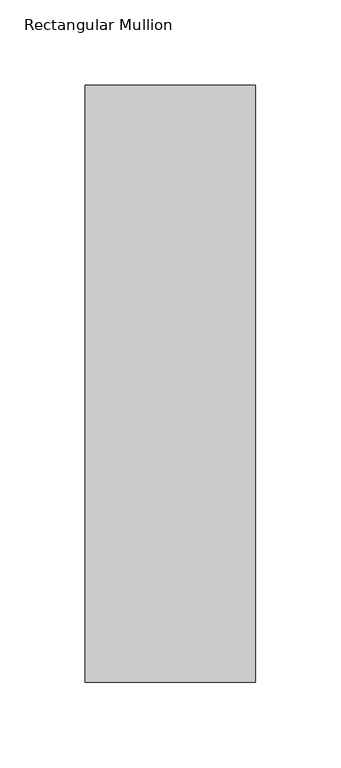
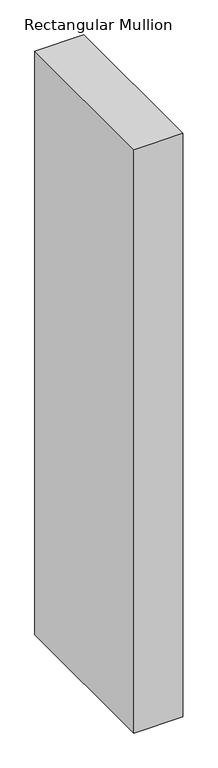
"""IFC4 building model written with IfcOpenShell, lengths in millimetres: member geometry, Rectangular Mullion : WWm-100x350-100mmOffset."""

import ifcopenshell
import ifcopenshell.guid

model = None  # the IFC model being written
_history = None  # IfcOwnerHistory: only IFC2X3 demands one
_inside = {}  # id of a spatial element -> (the spatial element, [elements in it])
_under = {}  # id of a project, library or spatial element -> (it, [spatial elements below it])
_declared = {}  # id of a project -> (the project, [libraries it declares])
_typed = {}  # id of a type object -> (the type object, [elements of that type])
_made_of = {}  # id of a material, layer set ... -> (it, [elements and type objects made of it])


def new_model(schema):
    """Start an empty IFC model of exactly this schema.

    Asked for "IFC4X3", IfcOpenShell would pick the latest addendum, in which some entities
    have other attributes; the version numbers below select the first issue.
    IFC2X3 requires an IfcOwnerHistory on every rooted entity: one is made here for all.
    """
    global model, _history
    if schema == "IFC4X3":
        model = ifcopenshell.file(schema_version=(4, 3, 0, 0))
    else:
        model = ifcopenshell.file(schema=schema)
    _inside.clear()
    _under.clear()
    _declared.clear()
    _typed.clear()
    _made_of.clear()
    _history = None
    if model.schema == "IFC2X3":
        org = make("IfcOrganization", Name="unknown")
        user = make(
            "IfcPersonAndOrganization",
            ThePerson=make("IfcPerson", FamilyName="unknown"),
            TheOrganization=org,
        )
        app = make(
            "IfcApplication",
            ApplicationDeveloper=org,
            Version="unknown",
            ApplicationFullName="unknown",
            ApplicationIdentifier="unknown",
        )
        _history = make(
            "IfcOwnerHistory",
            OwningUser=user,
            OwningApplication=app,
            ChangeAction="ADDED",
            CreationDate=0,
        )
    return model


def make(cls, **values):
    """One entity of the class cls with the attributes given. An attribute that is None is left unset."""
    return model.create_entity(
        cls, **{name: value for name, value in values.items() if value is not None}
    )


def rooted(cls, **values):
    """An entity with a GlobalId (a new one), such as an element, a storey or a relation."""
    return make(cls, GlobalId=ifcopenshell.guid.new(), OwnerHistory=_history, **values)


def si_unit(unit_type, name, prefix=None):
    """IfcSIUnit, for example si_unit("LENGTHUNIT", "METRE", prefix="MILLI")."""
    return make("IfcSIUnit", UnitType=unit_type, Prefix=prefix, Name=name)


def assignment(units):
    """IfcUnitAssignment: the units of a project."""
    return None if units is None else make("IfcUnitAssignment", Units=units)


def point(xyz):
    """IfcCartesianPoint."""
    return None if xyz is None else make("IfcCartesianPoint", Coordinates=xyz)


def direction(xyz):
    """IfcDirection."""
    return None if xyz is None else make("IfcDirection", DirectionRatios=xyz)


def frame(location, z_axis=None, x_axis=None):
    """IfcAxis2Placement3D, a coordinate frame: its origin and axes. An axis left out is left unset."""
    return make(
        "IfcAxis2Placement3D",
        Location=point(location),
        Axis=direction(z_axis),
        RefDirection=direction(x_axis),
    )


def origin():
    """The frame at (0, 0, 0) with its axes left unset."""
    return frame((0.0, 0.0, 0.0))


def place(relative_to, where):
    """IfcLocalPlacement: puts the frame where relative to a parent placement (None: the world)."""
    return make(
        "IfcLocalPlacement", PlacementRelTo=relative_to, RelativePlacement=where
    )


def context(
    kind, dimensions, precision=None, world=None, true_north=None, identifier=None
):
    """IfcGeometricRepresentationContext, for example the 3D "Model" context."""
    return make(
        "IfcGeometricRepresentationContext",
        ContextIdentifier=identifier,
        ContextType=kind,
        CoordinateSpaceDimension=dimensions,
        Precision=precision,
        WorldCoordinateSystem=world,
        TrueNorth=true_north,
    )


def project(units=None, contexts=None):
    """IfcProject with its units and contexts."""
    return rooted(
        "IfcProject",
        Name="project",
        RepresentationContexts=contexts,
        UnitsInContext=assignment(units),
    )


def spatial(cls, under=None, at=None, **own):
    """A site, building, storey or space (cls), placed at a placement, below another one or the project."""
    s = rooted(cls, ObjectPlacement=at, **own)
    if under is not None:
        _under.setdefault(under.id(), (under, []))[1].append(s)
    return s


def polyline(points):
    """IfcPolyline through the points."""
    return make("IfcPolyline", Points=[point(p) for p in points])


def outline(outer, holes=None, kind="AREA"):
    """IfcArbitraryClosedProfileDef: a profile drawn as a closed curve; with holes, ...WithVoids."""
    if holes is None:
        return make("IfcArbitraryClosedProfileDef", ProfileType=kind, OuterCurve=outer)
    return make(
        "IfcArbitraryProfileDefWithVoids",
        ProfileType=kind,
        OuterCurve=outer,
        InnerCurves=holes,
    )


def extrude(swept, where, along, depth):
    """IfcExtrudedAreaSolid: the profile swept, set in the frame where, extruded along a direction by depth."""
    return make(
        "IfcExtrudedAreaSolid",
        SweptArea=swept,
        Position=where,
        ExtrudedDirection=direction(along),
        Depth=depth,
    )


def shape(context_of_items, identifier, shape_type, items):
    """IfcShapeRepresentation: the items that make up one representation, for example the "Body"."""
    return make(
        "IfcShapeRepresentation",
        ContextOfItems=context_of_items,
        RepresentationIdentifier=identifier,
        RepresentationType=shape_type,
        Items=items,
    )


def source(mapping_origin, context_of_items, identifier, shape_type, items):
    """IfcRepresentationMap: a shape defined once, which mapped items show again and again."""
    return make(
        "IfcRepresentationMap",
        MappingOrigin=mapping_origin,
        MappedRepresentation=shape(context_of_items, identifier, shape_type, items),
    )


def transform(
    local_origin,
    x_axis=None,
    y_axis=None,
    z_axis=None,
    scale=None,
    scale2=None,
    scale3=None,
    uniform=True,
):
    """IfcCartesianTransformationOperator3D, or its non-uniform kind. x_axis, y_axis, z_axis: its Axis1, 2, 3."""
    if uniform:
        return make(
            "IfcCartesianTransformationOperator3D",
            Axis1=direction(x_axis),
            Axis2=direction(y_axis),
            LocalOrigin=point(local_origin),
            Scale=scale,
            Axis3=direction(z_axis),
        )
    return make(
        "IfcCartesianTransformationOperator3DnonUniform",
        Axis1=direction(x_axis),
        Axis2=direction(y_axis),
        LocalOrigin=point(local_origin),
        Scale=scale,
        Axis3=direction(z_axis),
        Scale2=scale2,
        Scale3=scale3,
    )


def mapped(mapping_source, mapping_target):
    """IfcMappedItem: shows the shape of a source again, moved by a transform."""
    return make(
        "IfcMappedItem", MappingSource=mapping_source, MappingTarget=mapping_target
    )


def made_of(thing, what):
    """Note that an element or type object is made of a material, layer set ...; save() writes the relation."""
    if what is not None:
        _made_of.setdefault(what.id(), (what, []))[1].append(thing)
    return thing


def element(
    cls,
    number,
    at=None,
    inside=None,
    cuts=None,
    type_object=None,
    material=None,
    context=None,
    identifier="Body",
    shape_type=None,
    held_by="IfcProductDefinitionShape",
    body=None,
    shapes=None,
    **own,
):
    """One element of the class cls, such as IfcWall. Its Tag is "e" and its number.

    at: its placement. inside: the storey or other place that contains it. cuts: it is an
    opening in that element (IfcRelVoidsElement). A single representation is given by context,
    identifier, shape_type and body (its items); several are given by shapes. held_by: the class
    of the entity that holds the representations. save() writes the other relations.
    """
    e = rooted(cls, Tag="e%d" % number, ObjectPlacement=at, **own)
    if body is not None:
        shapes = [shape(context, identifier, shape_type, body)]
    if shapes is not None:
        e.Representation = make(held_by, Representations=shapes)
    if inside is not None:
        _inside.setdefault(inside.id(), (inside, []))[1].append(e)
    if cuts is not None:
        rooted(
            "IfcRelVoidsElement", RelatingBuildingElement=cuts, RelatedOpeningElement=e
        )
    if type_object is not None:
        _typed.setdefault(type_object.id(), (type_object, []))[1].append(e)
    return made_of(e, material)


def aggregate(whole, parts):
    """IfcRelAggregates: a whole, such as a stair, and the parts it consists of."""
    return rooted("IfcRelAggregates", RelatingObject=whole, RelatedObjects=parts)


def save(model, path):
    """Write the relations noted so far, then the file.

    IfcRelAggregates (storeys below a building ...), IfcRelContainedInSpatialStructure (elements
    in a storey), IfcRelDefinesByType, IfcRelAssociatesMaterial and IfcRelDeclares: one each for
    every whole, place, type object, material and project.
    """
    for whole, parts in _under.values():
        aggregate(whole, parts)
    for where, things in _inside.values():
        rooted(
            "IfcRelContainedInSpatialStructure",
            RelatedElements=things,
            RelatingStructure=where,
        )
    for kind, things in _typed.values():
        rooted("IfcRelDefinesByType", RelatedObjects=things, RelatingType=kind)
    for what, things in _made_of.values():
        rooted("IfcRelAssociatesMaterial", RelatedObjects=things, RelatingMaterial=what)
    for by, libraries in _declared.values():
        rooted("IfcRelDeclares", RelatingContext=by, RelatedDefinitions=libraries)
    model.write(path)


def rectangular_mullion_8961ee6e(model_context):
    return source(origin(), model_context, "Body", "SweptSolid", [
        extrude(outline(polyline([(0.0, 175.0), (0.0, -175.0), (-100.0, -175.0), (-100.0, 175.0), (0.0, 175.0)])), frame((0.0, 0.0, -1258.3985335), z_axis=(0.0, 0.0, 1.0), x_axis=(1.0, 0.0, 0.0)), (0.0, 0.0, 1.0), 1258.3985335),
    ])


if __name__ == "__main__":
    model = new_model("IFC4")
    model_context = context("Model", 3, world=origin())
    ifc_project = project(units=[si_unit("LENGTHUNIT", "METRE", prefix="MILLI")], contexts=[model_context])
    site = spatial("IfcSite", under=ifc_project)
    building = spatial("IfcBuilding", under=site)
    placement = place(None, origin())
    rectangular_mullion_shape = rectangular_mullion_8961ee6e(model_context)
    element("IfcMember", 1, ObjectType="Rectangular Mullion : WWm-100x350-100mmOffset", at=placement, inside=building, context=model_context, shape_type="MappedRepresentation", body=[
        mapped(rectangular_mullion_shape, transform((0.0, 0.0, 0.0), x_axis=(1.0, 0.0, 0.0), y_axis=(0.0, 1.0, 0.0), z_axis=(0.0, 0.0, 1.0))),
    ])
    save(model, "model.ifc")

# Revit data of these elements
# Type "Rectangular Mullion : WWm-100x350-100mmOffset"
#   built-in parameter 1007304 = 1.14829 (stored number, unit not read)
#   built-in parameter 1007301 = 0.164042 (stored number, unit not read)
#   built-in parameter 1007300 = 0.164042 (stored number, unit not read)
# Element 1 (IfcMember, "Rectangular Mullion : WWm-100x350-100mmOffset")
#   Materials on its faces: "WW-EC-RGB-Mullion"
# Materials
#   "WW-EC-RGB-Mullion": class "Generic", colour RGB 255 255 255, transparency 0, Comments = "If region requests black mullions, switch asset color to RGB 25-25-25", Description = "Generic Color", Cost = 0
